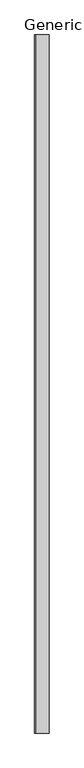
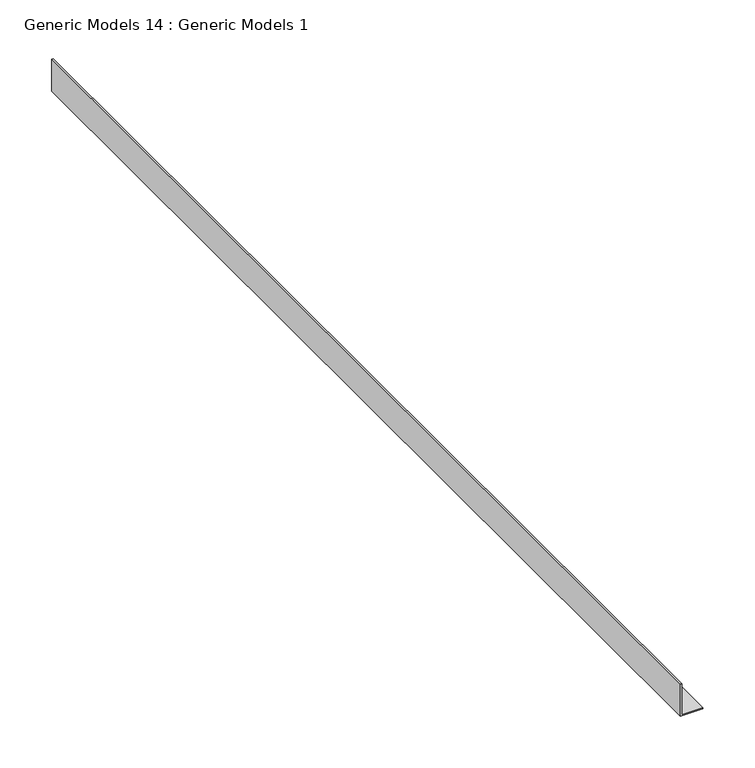
"""IFC4 building model written with IfcOpenShell, lengths in millimetres: proxy geometry, Generic Models 14 : Generic Models 1."""

from ifc_helpers import new_model, si_unit, frame, origin, place, context, project, spatial, polyline, outline, extrude, source, transform, mapped, element, save


def generic_models_14_generic_models_1_a3fd2df9(model_context):
    return source(origin(), model_context, "Body", "SweptSolid", [
        extrude(outline(polyline([(352.6731772, 52666.3196108), (314.5731772, 52666.3196108), (314.5731772, 52691.7196108), (316.1606772, 52691.7196108), (316.1606772, 52667.9071108), (352.6731772, 52667.9071108), (352.6731772, 52666.3196108)])), frame((0.0, 0.0, 0.0), z_axis=(0.0, 1.0, 0.0), x_axis=(0.0, 0.0, 1.0)), (0.0, 0.0, 1.0), 1219.2),
    ])


if __name__ == "__main__":
    model = new_model("IFC4")
    model_context = context("Model", 3, world=origin())
    ifc_project = project(units=[si_unit("LENGTHUNIT", "METRE", prefix="MILLI")], contexts=[model_context])
    site = spatial("IfcSite", under=ifc_project)
    building = spatial("IfcBuilding", under=site)
    placement = place(None, origin())
    generic_models_14_generic_models_1_shape = generic_models_14_generic_models_1_a3fd2df9(model_context)
    element("IfcBuildingElementProxy", 1, Name="Generic Models 14 : Generic Models 1", ObjectType="Generic Models 14 : Generic Models 1", at=placement, inside=building, context=model_context, shape_type="MappedRepresentation", body=[
        mapped(generic_models_14_generic_models_1_shape, transform((0.0, 0.0, 0.0), x_axis=(1.0, 0.0, 0.0), y_axis=(0.0, 1.0, 0.0), z_axis=(0.0, 0.0, 1.0))),
    ])
    save(model, "model.ifc")

# Revit data of these elements
# Element 1 (IfcBuildingElementProxy, "Generic Models 14 : Generic Models 1")
#   Materials on its faces: "CEILING TRACK AS SCHEDULED"
# Materials
#   "CEILING TRACK AS SCHEDULED": class "Unassigned", colour RGB 210 209 208, transparency 0, Keynote = "M05121300.02", Cost = 0
